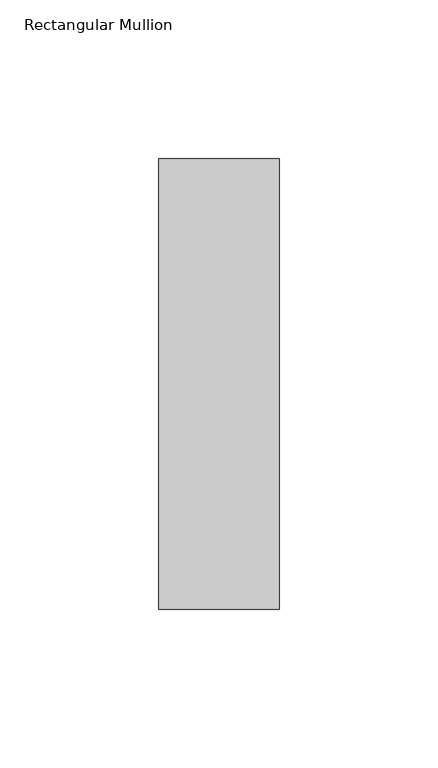
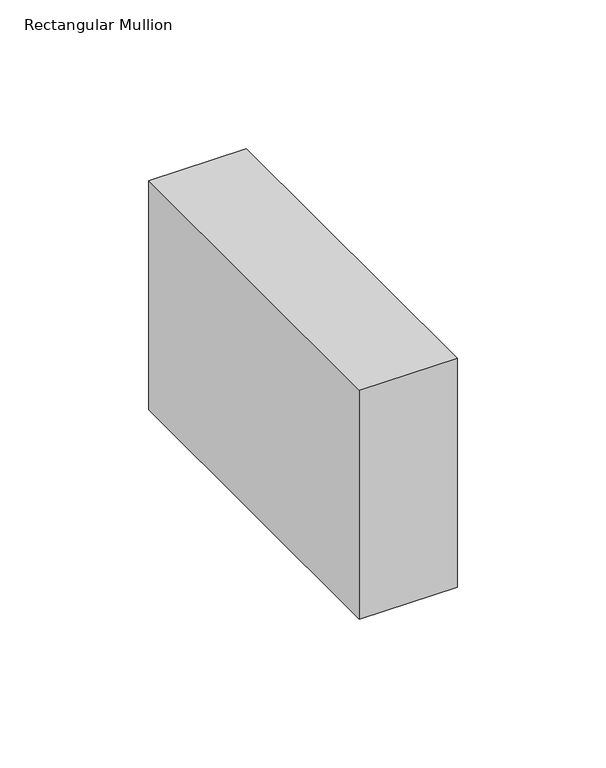
"""IFC4 building model written with IfcOpenShell, lengths in millimetres: member geometry, Rectangular Mullion : NLRS_21_CWM_hsb-regel 38x142_gen_rsf."""

from ifc_helpers import new_model, si_unit, frame, origin, place, context, project, spatial, polyline, outline, extrude, source, transform, mapped, element, save


def rectangular_mullion_06bc030d(model_context):
    return source(origin(), model_context, "Body", "SweptSolid", [
        extrude(outline(polyline([(19.0, -71.0), (-19.0, -71.0), (-19.0, 71.0), (19.0, 71.0), (19.0, -71.0)])), frame((0.0, 0.0, -94.1558939), z_axis=(0.0, 0.0, 1.0), x_axis=(1.0, 0.0, 0.0)), (0.0, 0.0, 1.0), 94.1558939),
    ])


if __name__ == "__main__":
    model = new_model("IFC4")
    model_context = context("Model", 3, world=origin())
    ifc_project = project(units=[si_unit("LENGTHUNIT", "METRE", prefix="MILLI")], contexts=[model_context])
    site = spatial("IfcSite", under=ifc_project)
    building = spatial("IfcBuilding", under=site)
    placement = place(None, origin())
    rectangular_mullion_shape = rectangular_mullion_06bc030d(model_context)
    element("IfcMember", 1, ObjectType="Rectangular Mullion : NLRS_21_CWM_hsb-regel 38x142_gen_rsf", at=placement, inside=building, context=model_context, shape_type="MappedRepresentation", body=[
        mapped(rectangular_mullion_shape, transform((0.0, 0.0, 0.0), x_axis=(1.0, 0.0, 0.0), y_axis=(0.0, 1.0, 0.0), z_axis=(0.0, 0.0, 1.0))),
    ])
    save(model, "model.ifc")

# Revit data of these elements
# Type "Rectangular Mullion : NLRS_21_CWM_hsb-regel 38x142_gen_rsf"
#   Export Type to IFC As = "IfcWall"
#   Type IfcGUID = "07M7mRoiH1CR8m_RSKIwpF"
#   Assembly Code = "21.10"
#   built-in parameter 1007322 = 0.465879 (stored number, unit not read)
#   built-in parameter 1007321 = 0.062336 (stored number, unit not read)
#   built-in parameter 1007320 = 0.062336 (stored number, unit not read)
# Element 1 (IfcMember, "Rectangular Mullion : NLRS_21_CWM_hsb-regel 38x142_gen_rsf")
#   Materials on its faces: "NLRS_i2_hout naaldhout vuren_gen_rsf"
# Materials
#   "NLRS_i2_hout naaldhout vuren_gen_rsf": class "I - Hout", colour RGB 234 199 147, transparency 0, Keynote = "i2", Manufacturer = "Revit Standards Foundation", URL = "www.revitstandards.org", Description = "hout vuren", Cost = 0
